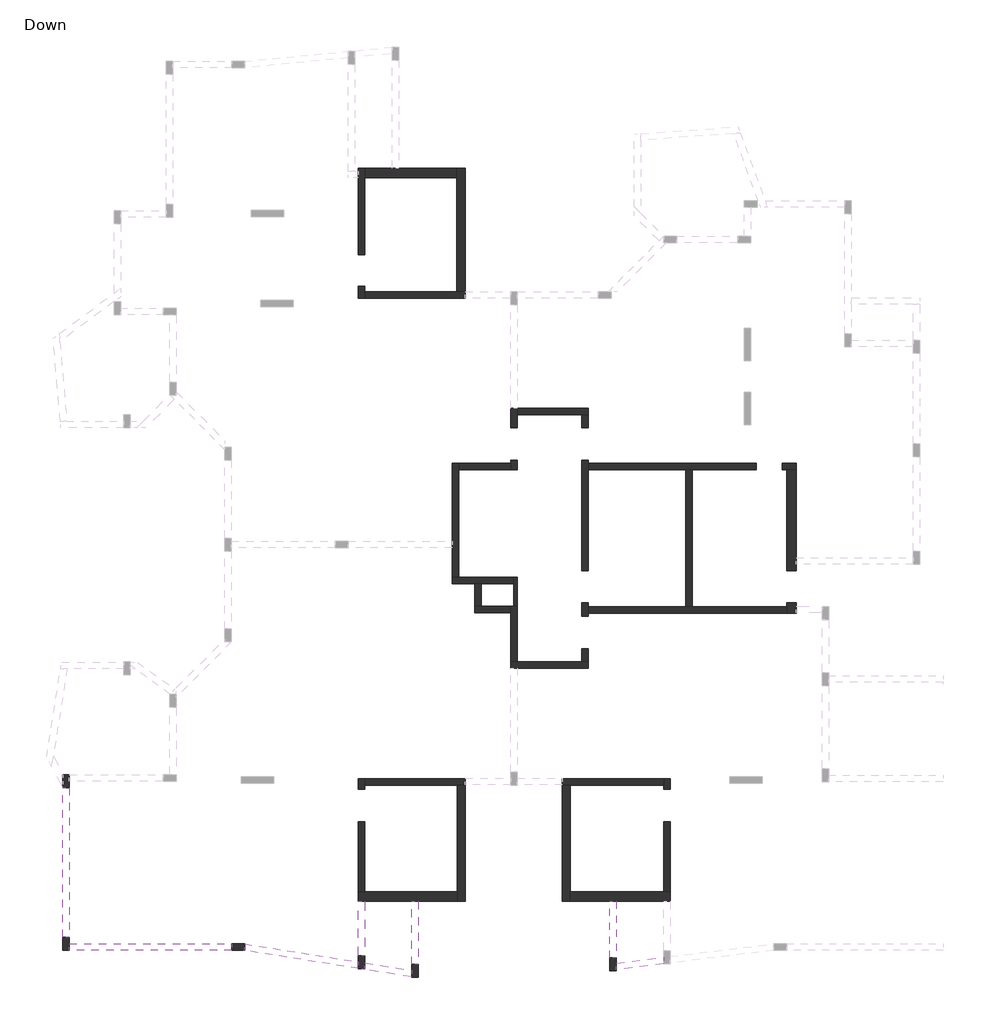
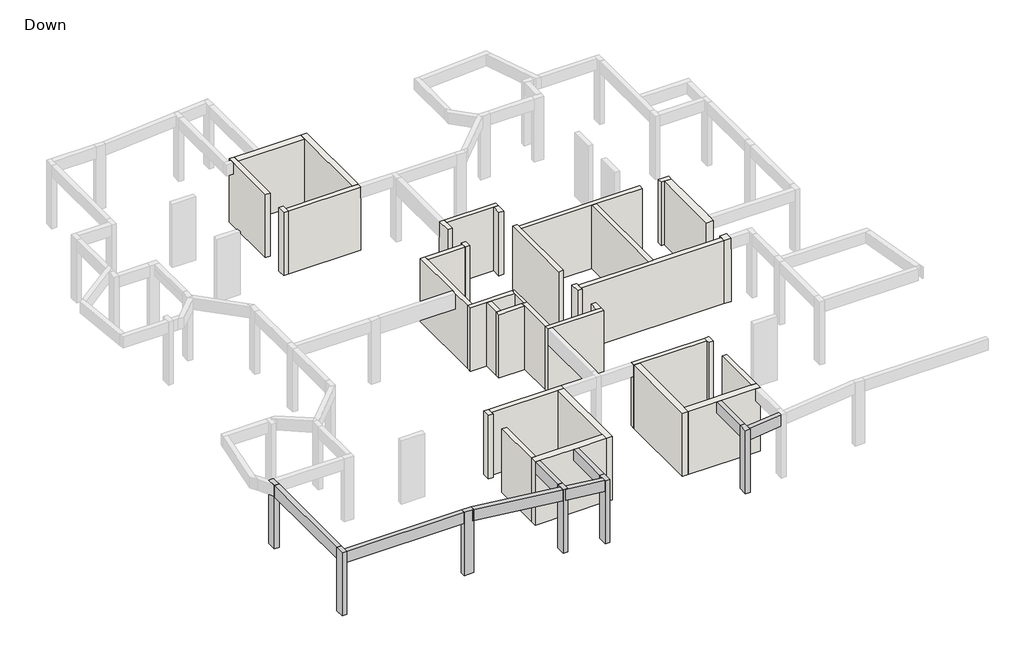
# One storey, part 1 of 3: 36 walls, 8 beams, 6 columns.
"""IFC4 building model written with IfcOpenShell, lengths in millimetres."""

from ifc_helpers import new_model, si_unit, frame, origin, place, context, project, spatial, polyline, outline, extrude, faceted_brep, element, save

model = new_model("IFC4")

# Units and contexts
model_context = context("Model", 3, world=origin())
ifc_project = project(units=[si_unit("LENGTHUNIT", "METRE", prefix="MILLI")], contexts=[model_context])

# Site, building, storey
site = spatial("IfcSite", under=ifc_project)
building = spatial("IfcBuilding", under=site)
storey = spatial("IfcBuildingStorey", under=building, Name="Down", Elevation=0.0)

# Beams
placement = place(None, origin())
element("IfcBeam", 1, ObjectType="Concrete Rectengular Beam : 20/50", at=placement, inside=storey, context=model_context, shape_type="Brep", body=[
    faceted_brep([(-9483.9897454, -17344.4159012, 2850.0), (-9283.9897454, -17344.4159012, 2850.0), (-9283.9897454, -15667.9244771, 2850.0), (-9483.9897454, -15667.9244771, 2850.0), (-9283.9897454, -17344.4159012, 2350.0), (-9283.9897454, -15667.9244771, 2350.0), (-9283.9897454, -15667.9244771, 2650.0), (-9483.9897454, -17344.4159012, 2350.0), (-9483.9897454, -15667.9244771, 2350.0), (-9483.9897454, -15667.9244771, 2650.0), (-9483.9897454, -17344.4159012, 2650.0)], [[[0, 1, 2, 3]], [[1, 4, 5, 6, 2]], [[4, 7, 8, 5]], [[0, 3, 9, 8, 7, 10]], [[1, 0, 10, 7, 4]], [[3, 2, 6, 5, 8, 9]]]),
])
element("IfcBeam", 2, ObjectType="Concrete Rectengular Beam : 20/50", at=placement, inside=storey, context=model_context, shape_type="Brep", body=[
    faceted_brep([(-9283.9897454, -17557.8098157, 2850.0), (-9283.9897454, -17744.4159012, 2850.0), (-9383.9897454, -17744.4159012, 2850.0), (-7844.4831614, -17989.3374032, 2850.0), (-7844.4831614, -17786.8222268, 2850.0), (-7844.4831614, -17786.8222268, 2650.0), (-7844.4831614, -17786.8222268, 2350.0), (-9283.9897454, -17557.8098157, 2350.0), (-9283.9897454, -17557.8098157, 2650.0), (-9283.9897454, -17744.4159012, 2350.0), (-7844.4831614, -17989.3374032, 2350.0), (-9383.9897454, -17744.4159012, 2350.0)], [[[0, 1, 2, 3, 4]], [[0, 4, 5, 6, 7, 8]], [[9, 7, 6, 10, 11]], [[2, 11, 10, 3]], [[9, 1, 0, 8, 7]], [[1, 9, 11, 2]], [[4, 3, 10, 6, 5]]]),
])
element("IfcBeam", 3, ObjectType="Concrete Rectengular Beam : 20/50", at=placement, inside=storey, context=model_context, shape_type="Brep", body=[
    faceted_brep([(-12973.5990213, -16973.3846199, 2850.0), (-12973.5990213, -17169.7313812, 2850.0), (-13012.4050044, -17169.7313812, 2850.0), (-9483.9897454, -17728.5774572, 2850.0), (-9483.9897454, -17526.0844321, 2850.0), (-9483.9897454, -17526.0844321, 2650.0), (-9483.9897454, -17526.0844321, 2350.0), (-12973.5990213, -16973.3846199, 2350.0), (-12973.5990213, -16973.3846199, 2650.0), (-12973.5990213, -17169.7313812, 2350.0), (-9483.9897454, -17728.5774572, 2350.0), (-13012.4050044, -17169.7313812, 2350.0)], [[[0, 1, 2, 3, 4]], [[0, 4, 5, 6, 7, 8]], [[9, 7, 6, 10, 11]], [[2, 11, 10, 3]], [[1, 9, 11, 2]], [[1, 0, 8, 7, 9]], [[3, 10, 6, 5, 4]]]),
])
element("IfcBeam", 4, ObjectType="Concrete Rectengular Beam : 20/50", at=placement, inside=storey, context=model_context, shape_type="Brep", body=[
    faceted_brep([(-18379.347479, -16969.7313812, 2850.0), (-18379.347479, -17169.7313812, 2850.0), (-13373.5990213, -17169.7313812, 2850.0), (-13373.5990213, -16969.7313812, 2850.0), (-13373.5990213, -16969.7313812, 2650.0), (-13373.5990213, -16969.7313812, 2350.0), (-18379.347479, -16969.7313812, 2350.0), (-18379.347479, -16969.7313812, 2650.0), (-18379.347479, -17169.7313812, 2350.0), (-13373.5990213, -17169.7313812, 2350.0)], [[[0, 1, 2, 3]], [[0, 3, 4, 5, 6, 7]], [[8, 6, 5, 9]], [[1, 8, 9, 2]], [[1, 0, 7, 6, 8]], [[3, 2, 9, 5, 4]]]),
])
element("IfcBeam", 5, ObjectType="Concrete Rectengular Beam : 20/50", at=placement, inside=storey, context=model_context, shape_type="Brep", body=[
    faceted_brep([(-7844.4831614, -17605.2464942, 2850.0), (-7644.4831614, -17605.2464942, 2850.0), (-7644.4831614, -15667.9244771, 2850.0), (-7844.4831614, -15667.9244771, 2850.0), (-7644.4831614, -17605.2464942, 2350.0), (-7644.4831614, -15667.9244771, 2350.0), (-7844.4831614, -17605.2464942, 2350.0), (-7844.4831614, -15667.9244771, 2350.0), (-7844.4831614, -15667.9244771, 2650.0)], [[[0, 1, 2, 3]], [[1, 4, 5, 2]], [[4, 6, 7, 5]], [[6, 0, 3, 8, 7]], [[1, 0, 6, 4]], [[3, 2, 5, 7, 8]]]),
])
element("IfcBeam", 6, ObjectType="Concrete Rectengular Beam : 20/50", at=placement, inside=storey, context=model_context, shape_type="SweptSolid", body=[
    extrude(outline(polyline([(-18579.347479, -12165.3513235), (-18379.347479, -12165.3513235), (-18379.347479, -16769.7313812), (-18579.347479, -16769.7313812), (-18579.347479, -12165.3513235)])), frame((0.0, 0.0, 2350.0), z_axis=(0.0, 0.0, 1.0), x_axis=(1.0, 0.0, 0.0)), (0.0, 0.0, 1.0), 500.0),
])
element("IfcBeam", 7, ObjectType="Concrete Rectengular Beam : 20/50", at=placement, inside=storey, context=model_context, shape_type="Brep", body=[
    faceted_brep([(-1546.410046, -17563.5051163, 2850.0), (-1546.410046, -17765.0070814, 2850.0), (-87.6035477, -17585.8881661, 2850.0), (-87.6035477, -17384.386201, 2850.0), (-87.6035477, -17384.386201, 2650.0), (-87.6035477, -17384.386201, 2350.0), (-1546.410046, -17563.5051163, 2350.0), (-1546.410046, -17563.5051163, 2650.0), (-1546.410046, -17765.0070814, 2350.0), (-87.6035477, -17585.8881661, 2350.0)], [[[0, 1, 2, 3]], [[0, 3, 4, 5, 6, 7]], [[8, 6, 5, 9]], [[1, 8, 9, 2]], [[1, 0, 7, 6, 8]], [[3, 2, 9, 5, 4]]]),
])
element("IfcBeam", 8, ObjectType="Concrete Rectengular Beam : 20/50", at=placement, inside=storey, context=model_context, shape_type="Brep", body=[
    faceted_brep([(-1746.410046, -17401.7807651, 2850.0), (-1546.410046, -17401.7807651, 2850.0), (-1546.410046, -15667.9244771, 2850.0), (-1746.410046, -15667.9244771, 2850.0), (-1546.410046, -17401.7807651, 2350.0), (-1546.410046, -15667.9244771, 2350.0), (-1546.410046, -15667.9244771, 2650.0), (-1746.410046, -17401.7807651, 2350.0), (-1746.410046, -15667.9244771, 2350.0)], [[[0, 1, 2, 3]], [[1, 4, 5, 6, 2]], [[4, 7, 8, 5]], [[7, 0, 3, 8]], [[1, 0, 7, 4]], [[3, 2, 6, 5, 8]]]),
])

# Columns
element("IfcColumn", 9, ObjectType="Concrete Rectengular Column : 20/40", at=placement, inside=storey, context=model_context, shape_type="Brep", body=[
    faceted_brep([(-18379.347479, -11765.3513235, 0.0), (-18379.347479, -12165.3513235, 0.0), (-18579.347479, -12165.3513235, 0.0), (-18579.347479, -11765.3513235, 0.0), (-18379.347479, -11765.3513235, 2850.0), (-18379.347479, -11965.3513235, 2850.0), (-18379.347479, -12165.3513235, 2850.0), (-18579.347479, -12165.3513235, 2850.0), (-18579.347479, -12157.819908, 2850.0), (-18579.347479, -11765.3513235, 2850.0), (-18579.347479, -11765.3513235, 2350.0), (-18561.5127169, -11765.3513235, 2850.0)], [[[0, 1, 2, 3]], [[4, 5, 6, 1, 0]], [[6, 7, 2, 1]], [[7, 8, 9, 10, 3, 2]], [[9, 11, 4, 0, 3, 10]], [[4, 11, 9, 8, 7, 6, 5]]]),
])
element("IfcColumn", 10, ObjectType="Concrete Rectengular Column : 20/40", at=placement, inside=storey, context=model_context, shape_type="Brep", body=[
    faceted_brep([(-18579.347479, -17169.7313812, 0.0), (-18579.347479, -16769.7313812, 0.0), (-18379.347479, -16769.7313812, 0.0), (-18379.347479, -17169.7313812, 0.0), (-18579.347479, -17169.7313812, 2850.0), (-18579.347479, -16769.7313812, 2850.0), (-18379.347479, -16769.7313812, 2850.0), (-18379.347479, -16969.7313812, 2850.0), (-18379.347479, -17169.7313812, 2850.0)], [[[0, 1, 2, 3]], [[4, 5, 1, 0]], [[5, 6, 2, 1]], [[6, 7, 8, 3, 2]], [[8, 4, 0, 3]], [[4, 8, 7, 6, 5]]]),
])
element("IfcColumn", 11, ObjectType="Concrete Rectengular Column : 20/40", at=placement, inside=storey, context=model_context, shape_type="Brep", body=[
    faceted_brep([(-12973.5990213, -17169.7313812, 0.0), (-13373.5990213, -17169.7313812, 0.0), (-13373.5990213, -16969.7313812, 0.0), (-12973.5990213, -16969.7313812, 0.0), (-12973.5990213, -17169.7313812, 2850.0), (-13373.5990213, -17169.7313812, 2850.0), (-13373.5990213, -16969.7313812, 2850.0), (-12973.5990213, -16969.7313812, 2850.0), (-12973.5990213, -16969.7313812, 2650.0), (-12973.5990213, -16973.3846199, 2850.0)], [[[0, 1, 2, 3]], [[4, 5, 1, 0]], [[5, 6, 2, 1]], [[6, 7, 8, 3, 2]], [[7, 9, 4, 0, 3, 8]], [[4, 9, 7, 6, 5]]]),
])
element("IfcColumn", 12, ObjectType="Concrete Rectengular Column : 20/40", at=placement, inside=storey, context=model_context, shape_type="Brep", body=[
    faceted_brep([(-9283.9897454, -17344.4159012, 0.0), (-9283.9897454, -17744.4159012, 0.0), (-9483.9897454, -17744.4159012, 0.0), (-9483.9897454, -17344.4159012, 0.0), (-9283.9897454, -17344.4159012, 2850.0), (-9283.9897454, -17557.8098157, 2850.0), (-9283.9897454, -17744.4159012, 2850.0), (-9483.9897454, -17744.4159012, 2850.0), (-9483.9897454, -17526.0844321, 2850.0), (-9483.9897454, -17344.4159012, 2850.0)], [[[0, 1, 2, 3]], [[4, 5, 6, 1, 0]], [[6, 7, 2, 1]], [[7, 8, 9, 3, 2]], [[9, 4, 0, 3]], [[4, 9, 8, 7, 6, 5]]]),
])
element("IfcColumn", 13, ObjectType="Concrete Rectengular Column : 20/40", at=placement, inside=storey, context=model_context, shape_type="Brep", body=[
    faceted_brep([(-7644.4831614, -17605.2464942, 0.0), (-7644.4831614, -18005.2464942, 0.0), (-7844.4831614, -18005.2464942, 0.0), (-7844.4831614, -17605.2464942, 0.0), (-7644.4831614, -17605.2464942, 2850.0), (-7644.4831614, -18005.2464942, 2850.0), (-7844.4831614, -18005.2464942, 2850.0), (-7844.4831614, -17786.8222268, 2850.0), (-7844.4831614, -17605.2464942, 2850.0)], [[[0, 1, 2, 3]], [[4, 5, 1, 0]], [[5, 6, 2, 1]], [[6, 7, 8, 3, 2]], [[8, 4, 0, 3]], [[4, 8, 7, 6, 5]]]),
])
element("IfcColumn", 14, ObjectType="Concrete Rectengular Column : 20/40", at=placement, inside=storey, context=model_context, shape_type="Brep", body=[
    faceted_brep([(-1546.410046, -17401.7807651, 0.0), (-1546.410046, -17801.7807651, 0.0), (-1746.410046, -17801.7807651, 0.0), (-1746.410046, -17401.7807651, 0.0), (-1546.410046, -17401.7807651, 2850.0), (-1546.410046, -17563.5051163, 2850.0), (-1546.410046, -17801.7807651, 2850.0), (-1746.410046, -17801.7807651, 2850.0), (-1746.410046, -17401.7807651, 2850.0)], [[[0, 1, 2, 3]], [[4, 5, 6, 1, 0]], [[6, 7, 2, 1]], [[7, 8, 3, 2]], [[8, 4, 0, 3]], [[4, 8, 7, 6, 5]]]),
])

# Walls
element("IfcWall", 15, ObjectType="10", at=placement, inside=storey, context=model_context, shape_type="Brep", body=[
    faceted_brep([(-4697.6379386, -5683.2914692, 0.0), (-4697.6379386, -5883.2914692, 0.0), (-4697.6379386, -6583.2914692, 0.0), (-4697.6379386, -6583.2914692, 2850.0), (-4697.6379386, -5883.2914692, 2850.0), (-4697.6379386, -5683.2914692, 2850.0), (-4597.6379386, -5683.2914692, 0.0), (-4597.6379386, -5683.2914692, 2650.0), (-4597.6379386, -5683.2914692, 2850.0), (-4597.6379386, -6583.2914692, 2850.0), (-4597.6379386, -6583.2914692, 0.0), (-4602.6379386, -5683.2914692, 2850.0)], [[[0, 1, 2, 3, 4, 5]], [[6, 7, 8, 9, 10]], [[2, 1, 0, 6, 10]], [[5, 4, 3, 9, 8, 11]], [[3, 2, 10, 9]], [[0, 5, 11, 8, 7, 6]]]),
])
element("IfcWall", 16, ObjectType="20", at=placement, inside=storey, context=model_context, shape_type="Brep", body=[
    faceted_brep([(-9490.6856227, 6897.8899275, 0.0), (-9490.6856227, 4237.8899275, 0.0), (-9490.6856227, 4237.8899275, 2650.0), (-9490.6856227, 4237.8899275, 2850.0), (-9490.6856227, 6598.9542002, 2850.0), (-9490.6856227, 6798.9542002, 2850.0), (-9490.6856227, 6897.8899275, 2850.0), (-9490.6856227, 6897.8899275, 2650.0), (-9290.6856227, 6897.8899275, 0.0), (-9290.6856227, 6897.8899275, 2850.0), (-9290.6856227, 6597.8899275, 2850.0), (-9290.6856227, 4237.8899275, 2850.0), (-9290.6856227, 4237.8899275, 2650.0), (-9290.6856227, 4237.8899275, 0.0), (-9290.6856227, 6597.8899275, 0.0)], [[[0, 1, 2, 3, 4, 5, 6, 7]], [[8, 9, 10, 11, 12, 13, 14]], [[1, 0, 8, 14, 13]], [[3, 2, 1, 13, 12, 11]], [[6, 5, 4, 3, 11, 10, 9]], [[0, 7, 6, 9, 8]]]),
])
element("IfcWall", 17, ObjectType="20", at=placement, inside=storey, context=model_context, shape_type="Brep", body=[
    faceted_brep([(-9490.6856227, 3262.2142639, 0.0), (-9490.6856227, 2895.9323955, 0.0), (-9490.6856227, 2895.9323955, 2650.0), (-9490.6856227, 2895.9323955, 2850.0), (-9490.6856227, 3262.2142639, 2850.0), (-9490.6856227, 3262.2142639, 2650.0), (-9290.6856227, 3262.2142639, 0.0), (-9290.6856227, 3262.2142639, 2650.0), (-9290.6856227, 3262.2142639, 2850.0), (-9290.6856227, 3095.9323955, 2850.0), (-9290.6856227, 2895.9323955, 2850.0), (-9290.6856227, 2895.9323955, 0.0), (-9290.6856227, 3095.9323955, 0.0)], [[[0, 1, 2, 3, 4, 5]], [[6, 7, 8, 9, 10, 11, 12]], [[1, 0, 6, 12, 11]], [[4, 3, 10, 9, 8]], [[0, 5, 4, 8, 7, 6]], [[3, 2, 1, 11, 10]]]),
])
element("IfcWall", 18, ObjectType="20", at=placement, inside=storey, context=model_context, shape_type="Brep", body=[
    faceted_brep([(-9290.6856227, 2895.9323955, 0.0), (-6200.1625371, 2895.9323955, 0.0), (-6200.1625371, 2895.9323955, 2350.0), (-6200.1625371, 2895.9323955, 2850.0), (-9290.6856227, 2895.9323955, 2850.0), (-9290.6856227, 3095.9323955, 0.0), (-9290.6856227, 3095.9323955, 2650.0), (-9290.6856227, 3095.9323955, 2850.0), (-6450.1625371, 3095.9323955, 2850.0), (-6200.1625371, 3095.9323955, 2850.0), (-6200.1625371, 3095.9323955, 2350.0), (-6200.1625371, 3095.9323955, 0.0), (-6450.1625371, 3095.9323955, 0.0)], [[[0, 1, 2, 3, 4]], [[5, 6, 7, 8, 9, 10, 11, 12]], [[1, 0, 5, 12, 11]], [[4, 3, 9, 8, 7]], [[0, 4, 7, 6, 5]], [[3, 2, 1, 11, 10, 9]]]),
])
element("IfcWall", 19, ObjectType="20", at=placement, inside=storey, context=model_context, shape_type="Brep", body=[
    faceted_brep([(-9283.9897454, -12214.5716558, 0.0), (-9283.9897454, -12083.2914692, 0.0), (-9283.9897454, -11883.2914692, 0.0), (-9283.9897454, -11883.2914692, 2850.0), (-9283.9897454, -12083.2914692, 2850.0), (-9283.9897454, -12214.5716558, 2850.0), (-9283.9897454, -12214.5716558, 2650.0), (-9483.9897454, -12214.5716558, 0.0), (-9483.9897454, -12214.5716558, 2650.0), (-9483.9897454, -12214.5716558, 2850.0), (-9483.9897454, -11883.2914692, 2850.0), (-9483.9897454, -11883.2914692, 2650.0), (-9483.9897454, -11883.2914692, 0.0)], [[[0, 1, 2, 3, 4, 5, 6]], [[7, 8, 9, 10, 11, 12]], [[2, 1, 0, 7, 12]], [[5, 4, 3, 10, 9]], [[0, 6, 5, 9, 8, 7]], [[3, 2, 12, 11, 10]]]),
])
element("IfcWall", 20, ObjectType="20", at=placement, inside=storey, context=model_context, shape_type="Brep", body=[
    faceted_brep([(-9283.9897454, -12083.2914692, 0.0), (-6440.6856227, -12083.2914692, 0.0), (-6190.6856227, -12083.2914692, 0.0), (-6190.6856227, -12083.2914692, 2350.0), (-6190.6856227, -12083.2914692, 2850.0), (-6440.6856227, -12083.2914692, 2850.0), (-9283.9897454, -12083.2914692, 2850.0), (-9283.9897454, -12083.2914692, 2650.0), (-9283.9897454, -11883.2914692, 0.0), (-9283.9897454, -11883.2914692, 2850.0), (-6190.6856227, -11883.2914692, 2850.0), (-6190.6856227, -11883.2914692, 2350.0), (-6190.6856227, -11883.2914692, 0.0)], [[[0, 1, 2, 3, 4, 5, 6, 7]], [[8, 9, 10, 11, 12]], [[2, 1, 0, 8, 12]], [[6, 5, 4, 10, 9]], [[0, 7, 6, 9, 8]], [[4, 3, 2, 12, 11, 10]]]),
])
element("IfcWall", 21, ObjectType="20", at=placement, inside=storey, context=model_context, shape_type="Brep", body=[
    faceted_brep([(-9283.9897454, -15367.9244771, 0.0), (-9283.9897454, -13219.4691321, 0.0), (-9283.9897454, -13219.4691321, 2650.0), (-9283.9897454, -13219.4691321, 2850.0), (-9283.9897454, -15367.9244771, 2850.0), (-9283.9897454, -15367.9244771, 2650.0), (-9483.9897454, -15367.9244771, 0.0), (-9483.9897454, -15367.9244771, 2850.0), (-9483.9897454, -13219.4691321, 2850.0), (-9483.9897454, -13219.4691321, 2650.0), (-9483.9897454, -13219.4691321, 0.0)], [[[0, 1, 2, 3, 4, 5]], [[6, 7, 8, 9, 10]], [[1, 0, 6, 10]], [[3, 2, 1, 10, 9, 8]], [[4, 3, 8, 7]], [[0, 5, 4, 7, 6]]]),
])
element("IfcWall", 22, ObjectType="20", at=placement, inside=storey, context=model_context, shape_type="Brep", body=[
    faceted_brep([(112.3964523, -12214.5716558, 0.0), (112.3964523, -11883.2914692, 0.0), (112.3964523, -11883.2914692, 2650.0), (112.3964523, -11883.2914692, 2850.0), (112.3964523, -12214.5716558, 2850.0), (112.3964523, -12214.5716558, 2650.0), (-87.6035477, -12214.5716558, 0.0), (-87.6035477, -12214.5716558, 2650.0), (-87.6035477, -12214.5716558, 2850.0), (-87.6035477, -12083.2914692, 2850.0), (-87.6035477, -11883.2914692, 2850.0), (-87.6035477, -11883.2914692, 0.0), (-87.6035477, -12083.2914692, 0.0)], [[[0, 1, 2, 3, 4, 5]], [[6, 7, 8, 9, 10, 11, 12]], [[1, 0, 6, 12, 11]], [[4, 3, 10, 9, 8]], [[0, 5, 4, 8, 7, 6]], [[3, 2, 1, 11, 10]]]),
])
element("IfcWall", 23, ObjectType="20", at=placement, inside=storey, context=model_context, shape_type="Brep", body=[
    faceted_brep([(-87.6035477, -11883.2914692, 0.0), (-3204.5902544, -11883.2914692, 0.0), (-3204.5902544, -11883.2914692, 2350.0), (-3204.5902544, -11883.2914692, 2850.0), (-87.6035477, -11883.2914692, 2850.0), (-87.6035477, -12083.2914692, 0.0), (-87.6035477, -12083.2914692, 2650.0), (-87.6035477, -12083.2914692, 2850.0), (-2954.5902544, -12083.2914692, 2850.0), (-3204.5902544, -12083.2914692, 2850.0), (-3204.5902544, -12083.2914692, 2350.0), (-3204.5902544, -12083.2914692, 0.0), (-2954.5902544, -12083.2914692, 0.0)], [[[0, 1, 2, 3, 4]], [[5, 6, 7, 8, 9, 10, 11, 12]], [[1, 0, 5, 12, 11]], [[4, 3, 9, 8, 7]], [[0, 4, 7, 6, 5]], [[3, 2, 1, 11, 10, 9]]]),
])
element("IfcWall", 24, ObjectType="20", at=placement, inside=storey, context=model_context, shape_type="Brep", body=[
    faceted_brep([(112.3964523, -15367.9244771, 0.0), (112.3964523, -13219.4691321, 0.0), (112.3964523, -13219.4691321, 2650.0), (112.3964523, -13219.4691321, 2850.0), (112.3964523, -15367.9244771, 2850.0), (-87.6035477, -15367.9244771, 0.0), (-87.6035477, -15367.9244771, 2650.0), (-87.6035477, -15367.9244771, 2850.0), (-87.6035477, -13219.4691321, 2850.0), (-87.6035477, -13219.4691321, 2650.0), (-87.6035477, -13219.4691321, 0.0)], [[[0, 1, 2, 3, 4]], [[5, 6, 7, 8, 9, 10]], [[1, 0, 5, 10]], [[3, 2, 1, 10, 9, 8]], [[4, 3, 8, 7]], [[0, 4, 7, 6, 5]]]),
])
element("IfcWall", 25, ObjectType="20", at=placement, inside=storey, context=model_context, shape_type="Brep", body=[
    faceted_brep([(-4797.6379386, -8483.2914692, 0.0), (-2403.3824041, -8483.2914692, 0.0), (-2403.3824041, -8483.2914692, 2650.0), (-2403.3824041, -8483.2914692, 2850.0), (-4597.6379386, -8483.2914692, 2850.0), (-4797.6379386, -8483.2914692, 2850.0), (-4797.6379386, -8283.2914692, 0.0), (-4797.6379386, -8283.2914692, 2850.0), (-4597.6379386, -8283.2914692, 2850.0), (-2603.3824041, -8283.2914692, 2850.0), (-2403.3824041, -8283.2914692, 2850.0), (-2403.3824041, -8283.2914692, 0.0), (-2603.3824041, -8283.2914692, 0.0), (-4597.6379386, -8283.2914692, 0.0)], [[[0, 1, 2, 3, 4, 5]], [[6, 7, 8, 9, 10, 11, 12, 13]], [[1, 0, 6, 13, 12, 11]], [[5, 4, 3, 10, 9, 8, 7]], [[3, 2, 1, 11, 10]], [[0, 5, 7, 6]]]),
])
element("IfcWall", 26, ObjectType="20", at=placement, inside=storey, context=model_context, shape_type="Brep", body=[
    faceted_brep([(-2403.3824041, -8283.2914692, 0.0), (-2403.3824041, -7883.2914692, 0.0), (-2403.3824041, -7883.2914692, 2650.0), (-2403.3824041, -7883.2914692, 2850.0), (-2403.3824041, -8283.2914692, 2850.0), (-2603.3824041, -8283.2914692, 0.0), (-2603.3824041, -8283.2914692, 2650.0), (-2603.3824041, -8283.2914692, 2850.0), (-2603.3824041, -7883.2914692, 2850.0), (-2603.3824041, -7883.2914692, 2650.0), (-2603.3824041, -7883.2914692, 0.0)], [[[0, 1, 2, 3, 4]], [[5, 6, 7, 8, 9, 10]], [[1, 0, 5, 10]], [[3, 2, 1, 10, 9, 8]], [[4, 3, 8, 7]], [[0, 4, 7, 6, 5]]]),
])
element("IfcWall", 27, ObjectType="20", at=placement, inside=storey, context=model_context, shape_type="Brep", body=[
    faceted_brep([(-2403.3824041, -6894.6673257, 0.0), (-2403.3824041, -6790.494584, 0.0), (-2403.3824041, -6590.494584, 0.0), (-2403.3824041, -6474.6673257, 0.0), (-2403.3824041, -6474.6673257, 2650.0), (-2403.3824041, -6474.6673257, 2850.0), (-2403.3824041, -6590.494584, 2850.0), (-2403.3824041, -6790.494584, 2850.0), (-2403.3824041, -6894.6673257, 2850.0), (-2403.3824041, -6894.6673257, 2650.0), (-2603.3824041, -6894.6673257, 0.0), (-2603.3824041, -6894.6673257, 2650.0), (-2603.3824041, -6894.6673257, 2850.0), (-2603.3824041, -6474.6673257, 2850.0), (-2603.3824041, -6474.6673257, 2650.0), (-2603.3824041, -6474.6673257, 0.0)], [[[0, 1, 2, 3, 4, 5, 6, 7, 8, 9]], [[10, 11, 12, 13, 14, 15]], [[3, 2, 1, 0, 10, 15]], [[5, 4, 3, 15, 14, 13]], [[8, 7, 6, 5, 13, 12]], [[0, 9, 8, 12, 11, 10]]]),
])
element("IfcWall", 28, ObjectType="20", at=placement, inside=storey, context=model_context, shape_type="Brep", body=[
    faceted_brep([(-2403.3824041, -6790.494584, 0.0), (3696.1514357, -6790.494584, 0.0), (3696.1514357, -6790.494584, 2850.0), (-2403.3824041, -6790.494584, 2850.0), (-2403.3824041, -6790.494584, 2650.0), (-2403.3824041, -6590.494584, 0.0), (-2403.3824041, -6590.494584, 2850.0), (596.6175959, -6590.494584, 2850.0), (796.6175959, -6590.494584, 2850.0), (3696.1514357, -6590.494584, 2850.0), (3696.1514357, -6590.494584, 2650.0), (3696.1514357, -6590.494584, 0.0), (796.6175959, -6590.494584, 0.0), (596.6175959, -6590.494584, 0.0)], [[[0, 1, 2, 3, 4]], [[5, 6, 7, 8, 9, 10, 11, 12, 13]], [[1, 0, 5, 13, 12, 11]], [[3, 2, 9, 8, 7, 6]], [[0, 4, 3, 6, 5]], [[2, 1, 11, 10, 9]]]),
])
element("IfcWall", 29, ObjectType="20", at=placement, inside=storey, context=model_context, shape_type="Brep", body=[
    faceted_brep([(-4597.6379386, -8283.2914692, 0.0), (-4597.6379386, -6583.2914692, 0.0), (-4597.6379386, -6583.2914692, 2850.0), (-4597.6379386, -8283.2914692, 2850.0), (-4597.6379386, -8283.2914692, 2650.0), (-4797.6379386, -8283.2914692, 0.0), (-4797.6379386, -8283.2914692, 2850.0), (-4797.6379386, -6783.2914692, 2850.0), (-4797.6379386, -6583.2914692, 2850.0), (-4797.6379386, -6583.2914692, 0.0), (-4797.6379386, -6783.2914692, 0.0), (-4697.6379386, -6583.2914692, 0.0), (-4697.6379386, -6583.2914692, 2850.0)], [[[0, 1, 2, 3, 4]], [[5, 6, 7, 8, 9, 10]], [[1, 0, 5, 10, 9, 11]], [[3, 2, 12, 8, 7, 6]], [[0, 4, 3, 6, 5]], [[2, 1, 11, 9, 8, 12]]]),
])
element("IfcWall", 30, ObjectType="20", at=placement, inside=storey, context=model_context, shape_type="Brep", body=[
    faceted_brep([(-4797.6379386, -6583.2914692, 0.0), (-5697.6379386, -6583.2914692, 0.0), (-5897.6379386, -6583.2914692, 0.0), (-5897.6379386, -6583.2914692, 2850.0), (-5697.6379386, -6583.2914692, 2850.0), (-4797.6379386, -6583.2914692, 2850.0), (-4797.6379386, -6783.2914692, 0.0), (-4797.6379386, -6783.2914692, 2650.0), (-4797.6379386, -6783.2914692, 2850.0), (-5897.6379386, -6783.2914692, 2850.0), (-5897.6379386, -6783.2914692, 2650.0), (-5897.6379386, -6783.2914692, 0.0)], [[[0, 1, 2, 3, 4, 5]], [[6, 7, 8, 9, 10, 11]], [[2, 1, 0, 6, 11]], [[5, 4, 3, 9, 8]], [[0, 5, 8, 7, 6]], [[3, 2, 11, 10, 9]]]),
])
element("IfcWall", 31, ObjectType="20", at=placement, inside=storey, context=model_context, shape_type="Brep", body=[
    faceted_brep([(-5697.6379386, -6583.2914692, 0.0), (-5697.6379386, -5883.2914692, 0.0), (-5697.6379386, -5883.2914692, 2850.0), (-5697.6379386, -6583.2914692, 2850.0), (-5897.6379386, -6583.2914692, 0.0), (-5897.6379386, -6583.2914692, 2850.0), (-5897.6379386, -5883.2914692, 2850.0), (-5897.6379386, -5883.2914692, 2650.0), (-5897.6379386, -5883.2914692, 0.0)], [[[0, 1, 2, 3]], [[4, 5, 6, 7, 8]], [[1, 0, 4, 8]], [[3, 2, 6, 5]], [[0, 3, 5, 4]], [[2, 1, 8, 7, 6]]]),
])
element("IfcWall", 32, ObjectType="20", at=placement, inside=storey, context=model_context, shape_type="Brep", body=[
    faceted_brep([(-4697.6379386, -5683.2914692, 0.0), (-6397.6379386, -5683.2914692, 0.0), (-6597.6379386, -5683.2914692, 0.0), (-6597.6379386, -5683.2914692, 2850.0), (-6397.6379386, -5683.2914692, 2850.0), (-4697.6379386, -5683.2914692, 2850.0), (-4697.6379386, -5883.2914692, 0.0), (-4697.6379386, -5883.2914692, 2850.0), (-5697.6379386, -5883.2914692, 2850.0), (-5897.6379386, -5883.2914692, 2850.0), (-6597.6379386, -5883.2914692, 2850.0), (-6597.6379386, -5883.2914692, 2650.0), (-6597.6379386, -5883.2914692, 0.0), (-5897.6379386, -5883.2914692, 0.0), (-5697.6379386, -5883.2914692, 0.0)], [[[0, 1, 2, 3, 4, 5]], [[6, 7, 8, 9, 10, 11, 12, 13, 14]], [[2, 1, 0, 6, 14, 13, 12]], [[5, 4, 3, 10, 9, 8, 7]], [[3, 2, 12, 11, 10]], [[0, 5, 7, 6]]]),
])
element("IfcWall", 33, ObjectType="20", at=placement, inside=storey, context=model_context, shape_type="Brep", body=[
    faceted_brep([(-6397.6379386, -5683.2914692, 0.0), (-6397.6379386, -2383.2914692, 0.0), (-6397.6379386, -2183.2914692, 0.0), (-6397.6379386, -2183.2914692, 2850.0), (-6397.6379386, -2383.2914692, 2850.0), (-6397.6379386, -5683.2914692, 2850.0), (-6597.6379386, -5683.2914692, 0.0), (-6597.6379386, -5683.2914692, 2850.0), (-6597.6379386, -4787.4320305, 2850.0), (-6597.6379386, -4587.4320305, 2850.0), (-6597.6379386, -2183.2914692, 2850.0), (-6597.6379386, -2183.2914692, 2650.0), (-6597.6379386, -2183.2914692, 0.0)], [[[0, 1, 2, 3, 4, 5]], [[6, 7, 8, 9, 10, 11, 12]], [[2, 1, 0, 6, 12]], [[5, 4, 3, 10, 9, 8, 7]], [[0, 5, 7, 6]], [[3, 2, 12, 11, 10]]]),
])
element("IfcWall", 34, ObjectType="20", at=placement, inside=storey, context=model_context, shape_type="Brep", body=[
    faceted_brep([(-6397.6379386, -2383.2914692, 0.0), (-4797.6379386, -2383.2914692, 0.0), (-4797.6379386, -2383.2914692, 2850.0), (-6397.6379386, -2383.2914692, 2850.0), (-6397.6379386, -2183.2914692, 0.0), (-6397.6379386, -2183.2914692, 2850.0), (-4797.6379386, -2183.2914692, 2850.0), (-4797.6379386, -2183.2914692, 2650.0), (-4797.6379386, -2183.2914692, 0.0)], [[[0, 1, 2, 3]], [[4, 5, 6, 7, 8]], [[1, 0, 4, 8]], [[3, 2, 6, 5]], [[0, 3, 5, 4]], [[2, 1, 8, 7, 6]]]),
])
element("IfcWall", 35, ObjectType="20", at=placement, inside=storey, context=model_context, shape_type="Brep", body=[
    faceted_brep([(-4597.6379386, -2383.2914692, 0.0), (-4597.6379386, -2083.2914692, 0.0), (-4597.6379386, -2083.2914692, 2650.0), (-4597.6379386, -2083.2914692, 2850.0), (-4597.6379386, -2383.2914692, 2850.0), (-4597.6379386, -2383.2914692, 2650.0), (-4797.6379386, -2383.2914692, 0.0), (-4797.6379386, -2383.2914692, 2850.0), (-4797.6379386, -2183.2914692, 2850.0), (-4797.6379386, -2083.2914692, 2850.0), (-4797.6379386, -2083.2914692, 2650.0), (-4797.6379386, -2083.2914692, 0.0), (-4797.6379386, -2183.2914692, 0.0), (-4602.6379386, -2383.2914692, 2850.0)], [[[0, 1, 2, 3, 4, 5]], [[6, 7, 8, 9, 10, 11, 12]], [[1, 0, 6, 12, 11]], [[3, 2, 1, 11, 10, 9]], [[4, 3, 9, 8, 7, 13]], [[0, 5, 4, 13, 7, 6]]]),
])
element("IfcWall", 36, ObjectType="20", at=placement, inside=storey, context=model_context, shape_type="Brep", body=[
    faceted_brep([(-4597.6379386, -1083.2914692, 0.0), (-4597.6379386, -683.2914692, 0.0), (-4597.6379386, -483.2914692, 0.0), (-4597.6379386, -483.2914692, 2150.0), (-4597.6379386, -483.2914692, 2850.0), (-4597.6379386, -683.2914692, 2850.0), (-4597.6379386, -1083.2914692, 2850.0), (-4597.6379386, -1083.2914692, 2650.0), (-4797.6379386, -1083.2914692, 0.0), (-4797.6379386, -1083.2914692, 2650.0), (-4797.6379386, -1083.2914692, 2850.0), (-4797.6379386, -483.2914692, 2850.0), (-4797.6379386, -483.2914692, 2150.0), (-4797.6379386, -483.2914692, 0.0)], [[[0, 1, 2, 3, 4, 5, 6, 7]], [[8, 9, 10, 11, 12, 13]], [[2, 1, 0, 8, 13]], [[6, 5, 4, 11, 10]], [[0, 7, 6, 10, 9, 8]], [[4, 3, 2, 13, 12, 11]]]),
])
element("IfcWall", 37, ObjectType="20", at=placement, inside=storey, context=model_context, shape_type="Brep", body=[
    faceted_brep([(-4597.6379386, -683.2914692, 0.0), (-2603.3824041, -683.2914692, 0.0), (-2403.3824041, -683.2914692, 0.0), (-2403.3824041, -683.2914692, 2850.0), (-2603.3824041, -683.2914692, 2850.0), (-4597.6379386, -683.2914692, 2850.0), (-4597.6379386, -683.2914692, 2650.0), (-4597.6379386, -483.2914692, 0.0), (-4597.6379386, -483.2914692, 2650.0), (-4597.6379386, -483.2914692, 2850.0), (-2403.3824041, -483.2914692, 2850.0), (-2403.3824041, -483.2914692, 2650.0), (-2403.3824041, -483.2914692, 0.0)], [[[0, 1, 2, 3, 4, 5, 6]], [[7, 8, 9, 10, 11, 12]], [[2, 1, 0, 7, 12]], [[5, 4, 3, 10, 9]], [[0, 6, 5, 9, 8, 7]], [[3, 2, 12, 11, 10]]]),
])
element("IfcWall", 38, ObjectType="20", at=placement, inside=storey, context=model_context, shape_type="Brep", body=[
    faceted_brep([(-2603.3824041, -683.2914692, 0.0), (-2603.3824041, -1083.2914692, 0.0), (-2603.3824041, -1083.2914692, 2650.0), (-2603.3824041, -1083.2914692, 2850.0), (-2603.3824041, -683.2914692, 2850.0), (-2603.3824041, -683.2914692, 2650.0), (-2403.3824041, -683.2914692, 0.0), (-2403.3824041, -683.2914692, 2850.0), (-2403.3824041, -1083.2914692, 2850.0), (-2403.3824041, -1083.2914692, 2650.0), (-2403.3824041, -1083.2914692, 0.0)], [[[0, 1, 2, 3, 4, 5]], [[6, 7, 8, 9, 10]], [[1, 0, 6, 10]], [[3, 2, 1, 10, 9, 8]], [[4, 3, 8, 7]], [[0, 5, 4, 7, 6]]]),
])
element("IfcWall", 39, ObjectType="20", at=placement, inside=storey, context=model_context, shape_type="Brep", body=[
    faceted_brep([(-2603.3824041, -2086.1332064, 0.0), (-2603.3824041, -5486.1332064, 0.0), (-2603.3824041, -5486.1332064, 2650.0), (-2603.3824041, -5486.1332064, 2850.0), (-2603.3824041, -2086.1332064, 2850.0), (-2603.3824041, -2086.1332064, 2650.0), (-2403.3824041, -2086.1332064, 0.0), (-2403.3824041, -2086.1332064, 2650.0), (-2403.3824041, -2086.1332064, 2850.0), (-2403.3824041, -2186.1332064, 2850.0), (-2403.3824041, -2386.1332064, 2850.0), (-2403.3824041, -5486.1332064, 2850.0), (-2403.3824041, -5486.1332064, 2650.0), (-2403.3824041, -5486.1332064, 0.0), (-2403.3824041, -2386.1332064, 0.0), (-2403.3824041, -2186.1332064, 0.0)], [[[0, 1, 2, 3, 4, 5]], [[6, 7, 8, 9, 10, 11, 12, 13, 14, 15]], [[1, 0, 6, 15, 14, 13]], [[3, 2, 1, 13, 12, 11]], [[4, 3, 11, 10, 9, 8]], [[0, 5, 4, 8, 7, 6]]]),
])
element("IfcWall", 40, ObjectType="20", at=placement, inside=storey, context=model_context, shape_type="Brep", body=[
    faceted_brep([(-2403.3824041, -2386.1332064, 0.0), (596.6175959, -2386.1332064, 0.0), (796.6175959, -2386.1332064, 0.0), (2756.6175959, -2386.1332064, 0.0), (2756.6175959, -2386.1332064, 2650.0), (2756.6175959, -2386.1332064, 2850.0), (796.6175959, -2386.1332064, 2850.0), (596.6175959, -2386.1332064, 2850.0), (-2403.3824041, -2386.1332064, 2850.0), (-2403.3824041, -2186.1332064, 0.0), (-2403.3824041, -2186.1332064, 2650.0), (-2403.3824041, -2186.1332064, 2850.0), (2756.6175959, -2186.1332064, 2850.0), (2756.6175959, -2186.1332064, 2650.0), (2756.6175959, -2186.1332064, 0.0)], [[[0, 1, 2, 3, 4, 5, 6, 7, 8]], [[9, 10, 11, 12, 13, 14]], [[3, 2, 1, 0, 9, 14]], [[5, 4, 3, 14, 13, 12]], [[8, 7, 6, 5, 12, 11]], [[0, 8, 11, 10, 9]]]),
])
element("IfcWall", 41, ObjectType="20", at=placement, inside=storey, context=model_context, shape_type="Brep", body=[
    faceted_brep([(3556.6175959, -2386.1332064, 0.0), (3696.1514357, -2386.1332064, 0.0), (3996.1514357, -2386.1332064, 0.0), (3996.1514357, -2386.1332064, 2850.0), (3696.1514357, -2386.1332064, 2850.0), (3556.6175959, -2386.1332064, 2850.0), (3556.6175959, -2386.1332064, 2650.0), (3556.6175959, -2186.1332064, 0.0), (3556.6175959, -2186.1332064, 2650.0), (3556.6175959, -2186.1332064, 2850.0), (3996.1514357, -2186.1332064, 2850.0), (3996.1514357, -2186.1332064, 2650.0), (3996.1514357, -2186.1332064, 0.0)], [[[0, 1, 2, 3, 4, 5, 6]], [[7, 8, 9, 10, 11, 12]], [[2, 1, 0, 7, 12]], [[5, 4, 3, 10, 9]], [[0, 6, 5, 9, 8, 7]], [[3, 2, 12, 11, 10]]]),
])
element("IfcWall", 42, ObjectType="20", at=placement, inside=storey, context=model_context, shape_type="Brep", body=[
    faceted_brep([(596.6175959, -2386.1332064, 0.0), (596.6175959, -6590.494584, 0.0), (596.6175959, -6590.494584, 2850.0), (596.6175959, -2386.1332064, 2850.0), (796.6175959, -2386.1332064, 0.0), (796.6175959, -2386.1332064, 2650.0), (796.6175959, -2386.1332064, 2850.0), (796.6175959, -6590.494584, 2850.0), (796.6175959, -6590.494584, 2650.0), (796.6175959, -6590.494584, 0.0)], [[[0, 1, 2, 3]], [[4, 5, 6, 7, 8, 9]], [[1, 0, 4, 9]], [[3, 2, 7, 6]], [[2, 1, 9, 8, 7]], [[0, 3, 6, 5, 4]]]),
])
element("IfcWall", 43, ObjectType="25", at=placement, inside=storey, context=model_context, shape_type="Brep", body=[
    faceted_brep([(-6200.1625371, 3095.9323955, 0.0), (-6200.1625371, 6897.8899275, 0.0), (-6200.1625371, 6897.8899275, 2850.0), (-6200.1625371, 3095.9323955, 2850.0), (-6450.1625371, 3095.9323955, 0.0), (-6450.1625371, 3095.9323955, 2650.0), (-6450.1625371, 3095.9323955, 2850.0), (-6450.1625371, 6597.8899275, 2850.0), (-6450.1625371, 6897.8899275, 2850.0), (-6450.1625371, 6897.8899275, 0.0), (-6450.1625371, 6597.8899275, 0.0)], [[[0, 1, 2, 3]], [[4, 5, 6, 7, 8, 9, 10]], [[1, 0, 4, 10, 9]], [[3, 2, 8, 7, 6]], [[0, 3, 6, 5, 4]], [[2, 1, 9, 8]]]),
])
element("IfcWall", 44, ObjectType="25", at=placement, inside=storey, context=model_context, shape_type="Brep", body=[
    faceted_brep([(-6440.6856227, -12083.2914692, 0.0), (-6440.6856227, -15367.9244771, 0.0), (-6440.6856227, -15667.9244771, 0.0), (-6440.6856227, -15667.9244771, 2850.0), (-6440.6856227, -15367.9244771, 2850.0), (-6440.6856227, -12083.2914692, 2850.0), (-6440.6856227, -12083.2914692, 2650.0), (-6190.6856227, -12083.2914692, 0.0), (-6190.6856227, -12083.2914692, 2850.0), (-6190.6856227, -15667.9244771, 2850.0), (-6190.6856227, -15667.9244771, 0.0)], [[[0, 1, 2, 3, 4, 5, 6]], [[7, 8, 9, 10]], [[2, 1, 0, 7, 10]], [[5, 4, 3, 9, 8]], [[0, 6, 5, 8, 7]], [[3, 2, 10, 9]]]),
])
element("IfcWall", 45, ObjectType="25", at=placement, inside=storey, context=model_context, shape_type="Brep", body=[
    faceted_brep([(-3204.5902544, -12083.2914692, 0.0), (-3204.5902544, -15667.9244771, 0.0), (-3204.5902544, -15667.9244771, 2850.0), (-3204.5902544, -12083.2914692, 2850.0), (-2954.5902544, -12083.2914692, 0.0), (-2954.5902544, -12083.2914692, 2650.0), (-2954.5902544, -12083.2914692, 2850.0), (-2954.5902544, -15367.9244771, 2850.0), (-2954.5902544, -15667.9244771, 2850.0), (-2954.5902544, -15667.9244771, 0.0), (-2954.5902544, -15367.9244771, 0.0)], [[[0, 1, 2, 3]], [[4, 5, 6, 7, 8, 9, 10]], [[1, 0, 4, 10, 9]], [[3, 2, 8, 7, 6]], [[0, 3, 6, 5, 4]], [[2, 1, 9, 8]]]),
])
element("IfcWall", 46, ObjectType="30", at=placement, inside=storey, context=model_context, shape_type="Brep", body=[
    faceted_brep([(-6450.1625371, 6897.8899275, 0.0), (-9290.6856227, 6897.8899275, 0.0), (-9290.6856227, 6897.8899275, 2850.0), (-8437.0941181, 6897.8899275, 2850.0), (-6450.1625371, 6897.8899275, 2850.0), (-6450.1625371, 6597.8899275, 0.0), (-6450.1625371, 6597.8899275, 2650.0), (-6450.1625371, 6597.8899275, 2850.0), (-9290.6856227, 6597.8899275, 2850.0), (-9290.6856227, 6597.8899275, 2650.0), (-9290.6856227, 6597.8899275, 0.0)], [[[0, 1, 2, 3, 4]], [[5, 6, 7, 8, 9, 10]], [[1, 0, 5, 10]], [[4, 3, 2, 8, 7]], [[0, 4, 7, 6, 5]], [[2, 1, 10, 9, 8]]]),
])
element("IfcWall", 47, ObjectType="30", at=placement, inside=storey, context=model_context, shape_type="Brep", body=[
    faceted_brep([(-6440.6856227, -15367.9244771, 0.0), (-9283.9897454, -15367.9244771, 0.0), (-9483.9897454, -15367.9244771, 0.0), (-9483.9897454, -15367.9244771, 2850.0), (-9283.9897454, -15367.9244771, 2850.0), (-6440.6856227, -15367.9244771, 2850.0), (-6440.6856227, -15367.9244771, 2650.0), (-6440.6856227, -15667.9244771, 0.0), (-6440.6856227, -15667.9244771, 2850.0), (-7844.4831614, -15667.9244771, 2850.0), (-9283.9897454, -15667.9244771, 2850.0), (-9483.9897454, -15667.9244771, 2850.0), (-9483.9897454, -15667.9244771, 0.0)], [[[0, 1, 2, 3, 4, 5, 6]], [[7, 8, 9, 10, 11, 12]], [[2, 1, 0, 7, 12]], [[5, 4, 3, 11, 10, 9, 8]], [[0, 6, 5, 8, 7]], [[3, 2, 12, 11]]]),
])
element("IfcWall", 48, ObjectType="30", at=placement, inside=storey, context=model_context, shape_type="Brep", body=[
    faceted_brep([(-2954.5902544, -15667.9244771, 0.0), (112.3964523, -15667.9244771, 0.0), (112.3964523, -15667.9244771, 2350.0), (112.3964523, -15667.9244771, 2850.0), (-87.6035477, -15667.9244771, 2850.0), (-1546.410046, -15667.9244771, 2850.0), (-2954.5902544, -15667.9244771, 2850.0), (-2954.5902544, -15367.9244771, 0.0), (-2954.5902544, -15367.9244771, 2650.0), (-2954.5902544, -15367.9244771, 2850.0), (-87.6035477, -15367.9244771, 2850.0), (112.3964523, -15367.9244771, 2850.0), (112.3964523, -15367.9244771, 0.0), (-87.6035477, -15367.9244771, 0.0)], [[[0, 1, 2, 3, 4, 5, 6]], [[7, 8, 9, 10, 11, 12, 13]], [[1, 0, 7, 13, 12]], [[6, 5, 4, 3, 11, 10, 9]], [[0, 6, 9, 8, 7]], [[3, 2, 1, 12, 11]]]),
])
element("IfcWall", 49, ObjectType="30", at=placement, inside=storey, context=model_context, shape_type="Brep", body=[
    faceted_brep([(3696.1514357, -2386.1332064, 0.0), (3696.1514357, -5486.1332064, 0.0), (3696.1514357, -5486.1332064, 2650.0), (3696.1514357, -5486.1332064, 2850.0), (3696.1514357, -2386.1332064, 2850.0), (3696.1514357, -2386.1332064, 2650.0), (3996.1514357, -2386.1332064, 0.0), (3996.1514357, -2386.1332064, 2850.0), (3996.1514357, -5091.9879156, 2850.0), (3996.1514357, -5486.1332064, 2850.0), (3996.1514357, -5486.1332064, 2650.0), (3996.1514357, -5486.1332064, 0.0)], [[[0, 1, 2, 3, 4, 5]], [[6, 7, 8, 9, 10, 11]], [[1, 0, 6, 11]], [[3, 2, 1, 11, 10, 9]], [[4, 3, 9, 8, 7]], [[0, 5, 4, 7, 6]]]),
])
element("IfcWall", 50, ObjectType="30", at=placement, inside=storey, context=model_context, shape_type="Brep", body=[
    faceted_brep([(3696.1514357, -6470.494584, 0.0), (3696.1514357, -6590.494584, 0.0), (3696.1514357, -6790.494584, 0.0), (3696.1514357, -6790.494584, 2850.0), (3696.1514357, -6590.494584, 2850.0), (3696.1514357, -6470.494584, 2850.0), (3696.1514357, -6470.494584, 2650.0), (3996.1514357, -6470.494584, 0.0), (3996.1514357, -6470.494584, 2650.0), (3996.1514357, -6470.494584, 2850.0), (3996.1514357, -6590.494584, 2850.0), (3996.1514357, -6790.494584, 2850.0), (3996.1514357, -6790.494584, 2350.0), (3996.1514357, -6790.494584, 0.0)], [[[0, 1, 2, 3, 4, 5, 6]], [[7, 8, 9, 10, 11, 12, 13]], [[2, 1, 0, 7, 13]], [[5, 4, 3, 11, 10, 9]], [[0, 6, 5, 9, 8, 7]], [[3, 2, 13, 12, 11]]]),
])

save(model, "model.ifc")

# Revit data of these elements
# Project information
#   Project Issue Date = "Issue Date"
#   Project Status = "Project Status"
#   Client Name = "לקוח"
#   Project Address = "Enter address here"
#   Project Name = "Project 040"
#   Project Number = "מספר פרויקט"
# Type "Concrete Rectengular Beam : 20/50"
#   Length [instance default] = 152.4 cm
#   b = 20 cm
#   h = 50 cm
#   Structural Material [instance default] = Concrete
#   Assembly Code = ""
# Type "Concrete Rectengular Column : 20/40"
#   b = 20 cm
#   h = 40 cm
#   Structural Material [instance default] = Concrete
# Type "10"
#   Layers, outside or top first: 10 cm "Concrete" (function 1)
# Type "20"
#   Layers, outside or top first: 20 cm "Concrete" (function 1)
# Type "25"
#   Layers, outside or top first: 25 cm "Concrete" (function 1)
# Type "30"
#   Layers, outside or top first: 30 cm "Concrete" (function 1)
# Element 1 (IfcBeam, "Concrete Rectengular Beam : 20/50")
#   Comments = ""
#   Mark = "B1"
#   SOFiSTiK_AMG_Comments = ""
#   SOFiSTiK_AMG_Scheduled = yes
#   SOFiSTiK_AMG_Adjusted = yes
#   Structural Material = Concrete
#   Phase Created = New Construction
#   Materials on its faces: "Concrete"
# Element 2 (IfcBeam, "Concrete Rectengular Beam : 20/50")
#   Comments = ""
#   Mark = "B2"
#   SOFiSTiK_AMG_Comments = ""
#   SOFiSTiK_AMG_Scheduled = yes
#   SOFiSTiK_AMG_Adjusted = yes
#   Structural Material = Concrete
#   Phase Created = New Construction
#   Materials on its faces: "Concrete"
# Element 3 (IfcBeam, "Concrete Rectengular Beam : 20/50")
#   Comments = ""
#   Mark = "B3"
#   SOFiSTiK_AMG_Comments = ""
#   SOFiSTiK_AMG_Scheduled = yes
#   SOFiSTiK_AMG_Adjusted = yes
#   Structural Material = Concrete
#   Phase Created = New Construction
#   Materials on its faces: "Concrete"
# Element 4 (IfcBeam, "Concrete Rectengular Beam : 20/50")
#   Comments = ""
#   Mark = "B4"
#   SOFiSTiK_AMG_Comments = ""
#   SOFiSTiK_AMG_Scheduled = yes
#   SOFiSTiK_AMG_Adjusted = yes
#   Structural Material = Concrete
#   Phase Created = New Construction
#   Materials on its faces: "Concrete"
# Element 5 (IfcBeam, "Concrete Rectengular Beam : 20/50")
#   Comments = ""
#   Mark = "B5"
#   SOFiSTiK_AMG_Comments = ""
#   SOFiSTiK_AMG_Scheduled = yes
#   SOFiSTiK_AMG_Adjusted = yes
#   Structural Material = Concrete
#   Phase Created = New Construction
#   Materials on its faces: "Concrete"
# Element 6 (IfcBeam, "Concrete Rectengular Beam : 20/50")
#   Comments = ""
#   Mark = "B6"
#   SOFiSTiK_AMG_Comments = ""
#   SOFiSTiK_AMG_Scheduled = yes
#   SOFiSTiK_AMG_Adjusted = yes
#   Structural Material = Concrete
#   Phase Created = New Construction
#   Materials on its faces: "Concrete"
# Element 7 (IfcBeam, "Concrete Rectengular Beam : 20/50")
#   Comments = ""
#   Mark = "B62"
#   SOFiSTiK_AMG_Comments = ""
#   SOFiSTiK_AMG_Scheduled = yes
#   SOFiSTiK_AMG_Adjusted = yes
#   Structural Material = Concrete
#   Phase Created = New Construction
#   Materials on its faces: "Concrete"
# Element 8 (IfcBeam, "Concrete Rectengular Beam : 20/50")
#   Comments = ""
#   Mark = "B64"
#   SOFiSTiK_AMG_Comments = ""
#   SOFiSTiK_AMG_Scheduled = yes
#   SOFiSTiK_AMG_Adjusted = yes
#   Structural Material = Concrete
#   Phase Created = New Construction
#   Materials on its faces: "Concrete"
# Element 9 (IfcColumn, "Concrete Rectengular Column : 20/40")
#   Comments = ""
#   Mark = "C22"
#   SOFiSTiK_AMG_Comments = ""
#   SOFiSTiK_AMG_Scheduled = yes
#   SOFiSTiK_AMG_Adjusted = yes
#   Structural Material = Concrete
#   Phase Created = New Construction
#   Materials on its faces: "Concrete"
# Element 10 (IfcColumn, "Concrete Rectengular Column : 20/40")
#   Comments = ""
#   Mark = "C24"
#   SOFiSTiK_AMG_Comments = ""
#   SOFiSTiK_AMG_Scheduled = yes
#   SOFiSTiK_AMG_Adjusted = yes
#   Structural Material = Concrete
#   Phase Created = New Construction
#   Materials on its faces: "Concrete"
# Element 11 (IfcColumn, "Concrete Rectengular Column : 20/40")
#   Comments = ""
#   Mark = "C25"
#   SOFiSTiK_AMG_Comments = ""
#   SOFiSTiK_AMG_Scheduled = yes
#   SOFiSTiK_AMG_Adjusted = yes
#   Structural Material = Concrete
#   Phase Created = New Construction
#   Materials on its faces: "Concrete"
# Element 12 (IfcColumn, "Concrete Rectengular Column : 20/40")
#   Comments = ""
#   Mark = "C26"
#   SOFiSTiK_AMG_Comments = ""
#   SOFiSTiK_AMG_Scheduled = yes
#   SOFiSTiK_AMG_Adjusted = yes
#   Structural Material = Concrete
#   Phase Created = New Construction
#   Materials on its faces: "Concrete"
# Element 13 (IfcColumn, "Concrete Rectengular Column : 20/40")
#   Comments = ""
#   Mark = "C27"
#   SOFiSTiK_AMG_Comments = ""
#   SOFiSTiK_AMG_Scheduled = yes
#   SOFiSTiK_AMG_Adjusted = yes
#   Structural Material = Concrete
#   Phase Created = New Construction
#   Materials on its faces: "Concrete"
# Element 14 (IfcColumn, "Concrete Rectengular Column : 20/40")
#   Comments = ""
#   Mark = "C29"
#   SOFiSTiK_AMG_Comments = ""
#   SOFiSTiK_AMG_Scheduled = yes
#   SOFiSTiK_AMG_Adjusted = yes
#   Structural Material = Concrete
#   Phase Created = New Construction
#   Materials on its faces: "Concrete"
# Element 15 (IfcWall, "10")
#   Comments = ""
#   Mark = "W36"
#   SOFiSTiK_EdgeZones = "W37"
#   SOFiSTiK_AMG_Comments = "Too Narrow /"
#   Top Offset = 0 cm
#   Base Offset = 0 cm
#   wall height = 285 cm
#   SOFiSTiK_AMG_Scheduled = yes
#   SOFiSTiK_AMG_Adjusted = yes
#   Phase Created = New Construction
#   Base Constraint = Down
#   Top Constraint = Typical Floor
#   Materials on its faces: "Concrete"
# Element 16 (IfcWall, "20")
#   Comments = ""
#   Mark = "W1"
#   SOFiSTiK_EdgeZones = "W1"
#   SOFiSTiK_AMG_Comments = ""
#   Top Offset = 0 cm
#   Base Offset = 0 cm
#   wall height = 285 cm
#   SOFiSTiK_AMG_Scheduled = yes
#   SOFiSTiK_AMG_Adjusted = yes
#   Phase Created = New Construction
#   Base Constraint = Down
#   Top Constraint = Typical Floor
#   Materials on its faces: "Concrete"
# Element 17 (IfcWall, "20")
#   Comments = ""
#   Mark = "W2"
#   SOFiSTiK_EdgeZones = "W2"
#   SOFiSTiK_AMG_Comments = ""
#   Top Offset = 0 cm
#   Base Offset = 0 cm
#   wall height = 285 cm
#   SOFiSTiK_AMG_Scheduled = yes
#   SOFiSTiK_AMG_Adjusted = yes
#   Phase Created = New Construction
#   Base Constraint = Down
#   Top Constraint = Typical Floor
#   Materials on its faces: "Concrete"
# Element 18 (IfcWall, "20")
#   Comments = ""
#   Mark = "W3"
#   SOFiSTiK_EdgeZones = "W3"
#   SOFiSTiK_AMG_Comments = ""
#   Top Offset = 0 cm
#   Base Offset = 0 cm
#   wall height = 285 cm
#   SOFiSTiK_AMG_Scheduled = yes
#   SOFiSTiK_AMG_Adjusted = yes
#   Phase Created = New Construction
#   Base Constraint = Down
#   Top Constraint = Typical Floor
#   Materials on its faces: "Concrete"
# Element 19 (IfcWall, "20")
#   Comments = ""
#   Mark = "W4"
#   SOFiSTiK_EdgeZones = "W4"
#   SOFiSTiK_AMG_Comments = ""
#   Top Offset = 0 cm
#   Base Offset = 0 cm
#   wall height = 285 cm
#   SOFiSTiK_AMG_Scheduled = yes
#   SOFiSTiK_AMG_Adjusted = yes
#   Phase Created = New Construction
#   Base Constraint = Down
#   Top Constraint = Typical Floor
#   Materials on its faces: "Concrete"
# Element 20 (IfcWall, "20")
#   Comments = ""
#   Mark = "W5"
#   SOFiSTiK_EdgeZones = "W5"
#   SOFiSTiK_AMG_Comments = ""
#   Top Offset = 0 cm
#   Base Offset = 0 cm
#   wall height = 285 cm
#   SOFiSTiK_AMG_Scheduled = yes
#   SOFiSTiK_AMG_Adjusted = yes
#   Phase Created = New Construction
#   Base Constraint = Down
#   Top Constraint = Typical Floor
#   Materials on its faces: "Concrete"
# Element 21 (IfcWall, "20")
#   Comments = ""
#   Mark = "W6"
#   SOFiSTiK_EdgeZones = "W6"
#   SOFiSTiK_AMG_Comments = ""
#   Top Offset = 0 cm
#   Base Offset = 0 cm
#   wall height = 285 cm
#   SOFiSTiK_AMG_Scheduled = yes
#   SOFiSTiK_AMG_Adjusted = yes
#   Phase Created = New Construction
#   Base Constraint = Down
#   Top Constraint = Typical Floor
#   Materials on its faces: "Concrete"
# Element 22 (IfcWall, "20")
#   Comments = ""
#   Mark = "W7"
#   SOFiSTiK_EdgeZones = "W7"
#   SOFiSTiK_AMG_Comments = ""
#   Top Offset = 0 cm
#   Base Offset = 0 cm
#   wall height = 285 cm
#   SOFiSTiK_AMG_Scheduled = yes
#   SOFiSTiK_AMG_Adjusted = yes
#   Phase Created = New Construction
#   Base Constraint = Down
#   Top Constraint = Typical Floor
#   Materials on its faces: "Concrete"
# Element 23 (IfcWall, "20")
#   Comments = ""
#   Mark = "W8"
#   SOFiSTiK_EdgeZones = "W8"
#   SOFiSTiK_AMG_Comments = ""
#   Top Offset = 0 cm
#   Base Offset = 0 cm
#   wall height = 285 cm
#   SOFiSTiK_AMG_Scheduled = yes
#   SOFiSTiK_AMG_Adjusted = yes
#   Phase Created = New Construction
#   Base Constraint = Down
#   Top Constraint = Typical Floor
#   Materials on its faces: "Concrete"
# Element 24 (IfcWall, "20")
#   Comments = ""
#   Mark = "W9"
#   SOFiSTiK_EdgeZones = "W9"
#   SOFiSTiK_AMG_Comments = ""
#   Top Offset = 0 cm
#   Base Offset = 0 cm
#   wall height = 285 cm
#   SOFiSTiK_AMG_Scheduled = yes
#   SOFiSTiK_AMG_Adjusted = yes
#   Phase Created = New Construction
#   Base Constraint = Down
#   Top Constraint = Typical Floor
#   Materials on its faces: "Concrete"
# Element 25 (IfcWall, "20")
#   Comments = ""
#   Mark = "W10"
#   SOFiSTiK_EdgeZones = "W10"
#   SOFiSTiK_AMG_Comments = ""
#   Top Offset = 0 cm
#   Base Offset = 0 cm
#   wall height = 285 cm
#   SOFiSTiK_AMG_Scheduled = yes
#   SOFiSTiK_AMG_Adjusted = yes
#   Phase Created = New Construction
#   Base Constraint = Down
#   Top Constraint = Typical Floor
#   Materials on its faces: "Concrete"
# Element 26 (IfcWall, "20")
#   Comments = ""
#   Mark = "W11"
#   SOFiSTiK_EdgeZones = "W11"
#   SOFiSTiK_AMG_Comments = ""
#   Top Offset = 0 cm
#   Base Offset = 0 cm
#   wall height = 285 cm
#   SOFiSTiK_AMG_Scheduled = yes
#   SOFiSTiK_AMG_Adjusted = yes
#   Phase Created = New Construction
#   Base Constraint = Down
#   Top Constraint = Typical Floor
#   Materials on its faces: "Concrete"
# Element 27 (IfcWall, "20")
#   Comments = ""
#   Mark = "W12"
#   SOFiSTiK_EdgeZones = "W12"
#   SOFiSTiK_AMG_Comments = ""
#   Top Offset = 0 cm
#   Base Offset = 0 cm
#   wall height = 285 cm
#   SOFiSTiK_AMG_Scheduled = yes
#   SOFiSTiK_AMG_Adjusted = yes
#   Phase Created = New Construction
#   Base Constraint = Down
#   Top Constraint = Typical Floor
#   Materials on its faces: "Concrete"
# Element 28 (IfcWall, "20")
#   Comments = ""
#   Mark = "W13"
#   SOFiSTiK_EdgeZones = "W13"
#   SOFiSTiK_AMG_Comments = ""
#   Top Offset = 0 cm
#   Base Offset = 0 cm
#   wall height = 285 cm
#   SOFiSTiK_AMG_Scheduled = yes
#   SOFiSTiK_AMG_Adjusted = yes
#   Phase Created = New Construction
#   Base Constraint = Down
#   Top Constraint = Typical Floor
#   Materials on its faces: "Concrete"
# Element 29 (IfcWall, "20")
#   Comments = ""
#   Mark = "W14"
#   SOFiSTiK_EdgeZones = "W14"
#   SOFiSTiK_AMG_Comments = ""
#   Top Offset = 0 cm
#   Base Offset = 0 cm
#   wall height = 285 cm
#   SOFiSTiK_AMG_Scheduled = yes
#   SOFiSTiK_AMG_Adjusted = yes
#   Phase Created = New Construction
#   Base Constraint = Down
#   Top Constraint = Typical Floor
#   Materials on its faces: "Concrete"
# Element 30 (IfcWall, "20")
#   Comments = ""
#   Mark = "W15"
#   SOFiSTiK_EdgeZones = "W15"
#   SOFiSTiK_AMG_Comments = ""
#   Top Offset = 0 cm
#   Base Offset = 0 cm
#   wall height = 285 cm
#   SOFiSTiK_AMG_Scheduled = yes
#   SOFiSTiK_AMG_Adjusted = yes
#   Phase Created = New Construction
#   Base Constraint = Down
#   Top Constraint = Typical Floor
#   Materials on its faces: "Concrete"
# Element 31 (IfcWall, "20")
#   Comments = ""
#   Mark = "W16"
#   SOFiSTiK_EdgeZones = "W16"
#   SOFiSTiK_AMG_Comments = ""
#   Top Offset = 0 cm
#   Base Offset = 0 cm
#   wall height = 285 cm
#   SOFiSTiK_AMG_Scheduled = yes
#   SOFiSTiK_AMG_Adjusted = yes
#   Phase Created = New Construction
#   Base Constraint = Down
#   Top Constraint = Typical Floor
#   Materials on its faces: "Concrete"
# Element 32 (IfcWall, "20")
#   Comments = ""
#   Mark = "W17"
#   SOFiSTiK_EdgeZones = "W17"
#   SOFiSTiK_AMG_Comments = ""
#   Top Offset = 0 cm
#   Base Offset = 0 cm
#   wall height = 285 cm
#   SOFiSTiK_AMG_Scheduled = yes
#   SOFiSTiK_AMG_Adjusted = yes
#   Phase Created = New Construction
#   Base Constraint = Down
#   Top Constraint = Typical Floor
#   Materials on its faces: "Concrete"
# Element 33 (IfcWall, "20")
#   Comments = ""
#   Mark = "W18"
#   SOFiSTiK_EdgeZones = "W19"
#   SOFiSTiK_AMG_Comments = ""
#   Top Offset = 0 cm
#   Base Offset = 0 cm
#   wall height = 285 cm
#   SOFiSTiK_AMG_Scheduled = yes
#   SOFiSTiK_AMG_Adjusted = yes
#   Phase Created = New Construction
#   Base Constraint = Down
#   Top Constraint = Typical Floor
